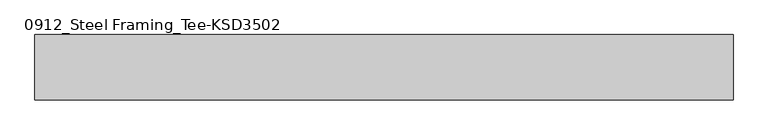
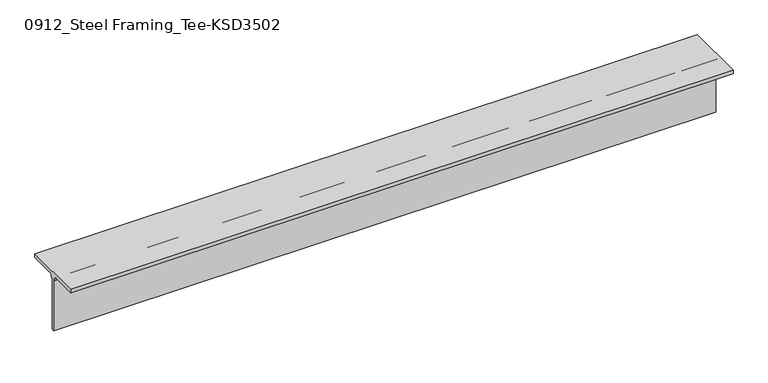
"""IFC4 building model written with IfcOpenShell, lengths in millimetres: member geometry, 0912_Steel Framing_Tee-KSD3502 : H_SB_ASB_CT-150x150x6.5x9."""

from ifc_helpers import new_model, si_unit, point, frame, frame_2d, origin, place, context, project, spatial, polyline, circle_curve, trimmed, segment, composite_curve, outline, extrude, source, transform, mapped, element, save


def member_0912_steel_framing_tee_ksd3502_a4b45e2e(model_context):
    return source(origin(), model_context, "Body", "SweptSolid", [
        extrude(outline(composite_curve([segment(polyline([(-75.0, 75.0), (75.0, 75.0), (75.0, 66.0), (16.25, 66.0)]), True, "CONTINUOUS"), segment(trimmed(circle_curve(frame_2d((16.25, 53.0)), 13.0), [point((16.25, 66.0))], [point((3.25, 53.0))], True, "CARTESIAN"), True, "CONTINUOUS"), segment(polyline([(3.25, 53.0), (3.25, -75.0), (-3.25, -75.0), (-3.25, 53.0)]), True, "CONTINUOUS"), segment(trimmed(circle_curve(frame_2d((-16.25, 53.0)), 13.0), [point((-3.25, 53.0))], [point((-16.25, 66.0))], True, "CARTESIAN"), True, "CONTINUOUS"), segment(polyline([(-16.25, 66.0), (-75.0, 66.0), (-75.0, 75.0)]), True, "CONTINUOUS")], self_intersect=False)), frame((-619.85, 0.0, 0.0), z_axis=(1.0, 0.0, 0.0), x_axis=(0.0, 1.0, 0.0)), (0.0, 0.0, 1.0), 1603.8),
    ])


if __name__ == "__main__":
    model = new_model("IFC4")
    model_context = context("Model", 3, world=origin())
    ifc_project = project(units=[si_unit("LENGTHUNIT", "METRE", prefix="MILLI")], contexts=[model_context])
    site = spatial("IfcSite", under=ifc_project)
    building = spatial("IfcBuilding", under=site)
    placement = place(None, origin())
    member_0912_steel_framing_tee_ksd3502_shape = member_0912_steel_framing_tee_ksd3502_a4b45e2e(model_context)
    element("IfcMember", 1, ObjectType="0912_Steel Framing_Tee-KSD3502 : H_SB_ASB_CT-150x150x6.5x9", at=placement, inside=building, context=model_context, shape_type="MappedRepresentation", body=[
        mapped(member_0912_steel_framing_tee_ksd3502_shape, transform((0.0, 0.0, 0.0), x_axis=(1.0, 0.0, 0.0), y_axis=(0.0, 1.0, 0.0), z_axis=(0.0, 0.0, 1.0))),
    ])
    save(model, "model.ifc")

# Revit data of these elements
# Type "0912_Steel Framing_Tee-KSD3502 : H_SB_ASB_CT-150x150x6.5x9"
#   H_WM Code_1 = "S01AA003-00001 | Main Steel Structure Fabrication Work | Shelter/Building | Light Steel - Standard (30KG/M>Weight) | Material: (   )"
#   H_WM Code_2 = "S03AA029-00001 | Main Steel Structure Erection Work | Shelter/Building | Light Steel (30KG/M>Weight) | Material: (   )"
#   H_WM Code_3 = "S01AA010-00001 | Main Steel Structure Fabrication Work | Shelter/Building | Steel Painting/Coating | for Non-Fireproofed Steel Surface, Surface Preparation, Primer, Second & Final Coat | Material: (   )"
#   H_Q'ty Cal Type Tag = "SB-Q2"
#   Width = 15.0 cm
#   Web Thickness = 0.65 cm
#   Web Fillet = 1.3 cm
#   Section Area = 23.39 cm²
#   Perimeter = 0.60 m²/m
#   Nominal Weight = 18.40 kgf/m
#   Height = 15.0 cm
#   Flange Thickness = 0.9 cm
#   Centroid Vertical = 7.5 cm
#   Centroid Horizontal = 7.5 cm
#   Length [instance default] = 1.5000 m
#   Structural Material [instance default] = Steel, 45-345
#   Warping Constant = (empty or 0)
#   Torsional Moment of Inertia = 0
#   Section Name Key = ""
#   Plastic Modulus weak axis = 0
#   Plastic Modulus strong axis = 0
#   Moment of Inertia weak axis = 0
#   Moment of Inertia strong axis = 0
#   Elastic Modulus weak axis = 0
#   Elastic Modulus strong axis = 0
#   Bolt Spacing = 0
#   Assembly Code = ""
# Element 1 (IfcMember, "0912_Steel Framing_Tee-KSD3502 : H_SB_ASB_CT-150x150x6.5x9")
#   Structural Material = none
# Materials
#   "Steel, 45-345": class "Metal", colour RGB 189 187 185, transparency 0, Description = "Steel 345 MPa", Cost = 0
